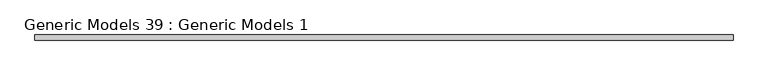
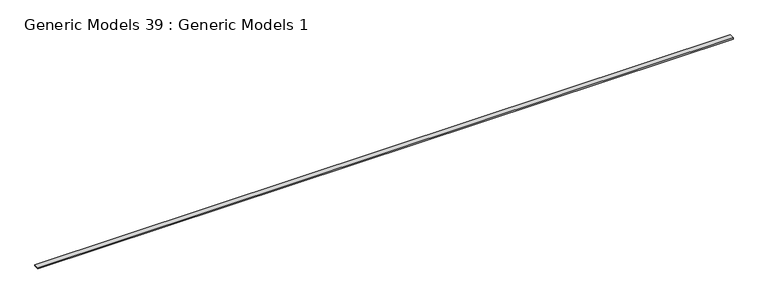
"""IFC4 building model written with IfcOpenShell, lengths in millimetres: proxy geometry, Generic Models 39 : Generic Models 1."""

from ifc_helpers import new_model, si_unit, frame, origin, place, context, project, spatial, polyline, outline, extrude, source, transform, mapped, element, save


def generic_models_39_generic_models_1_cf758188(model_context):
    return source(origin(), model_context, "Body", "SweptSolid", [
        extrude(outline(polyline([(-20998.9733045, 14098.1475835), (-20998.9733045, 14237.8475835), (-1948.9733045, 14237.8475835), (-1948.9733045, 14098.1475835), (-20998.9733045, 14098.1475835)])), frame((0.0, 0.0, 127066.3735933), z_axis=(0.0, 0.0, 1.0), x_axis=(1.0, 0.0, 0.0)), (0.0, 0.0, 1.0), 38.1),
    ])


if __name__ == "__main__":
    model = new_model("IFC4")
    model_context = context("Model", 3, world=origin())
    ifc_project = project(units=[si_unit("LENGTHUNIT", "METRE", prefix="MILLI")], contexts=[model_context])
    site = spatial("IfcSite", under=ifc_project)
    building = spatial("IfcBuilding", under=site)
    placement = place(None, origin())
    generic_models_39_generic_models_1_shape = generic_models_39_generic_models_1_cf758188(model_context)
    element("IfcBuildingElementProxy", 1, Name="Generic Models 39 : Generic Models 1", ObjectType="Generic Models 39 : Generic Models 1", at=placement, inside=building, context=model_context, shape_type="MappedRepresentation", body=[
        mapped(generic_models_39_generic_models_1_shape, transform((0.0, 0.0, 0.0), x_axis=(1.0, 0.0, 0.0), y_axis=(0.0, 1.0, 0.0), z_axis=(0.0, 0.0, 1.0))),
    ])
    save(model, "model.ifc")

# Revit data of these elements
# Element 1 (IfcBuildingElementProxy, "Generic Models 39 : Generic Models 1")
#   Materials on its faces: "_2X BLOCKING AS REQUIRED"
# Materials
#   "_2X BLOCKING AS REQUIRED": class "Generic", colour RGB 177 130 114, transparency 0, Cost = 0
